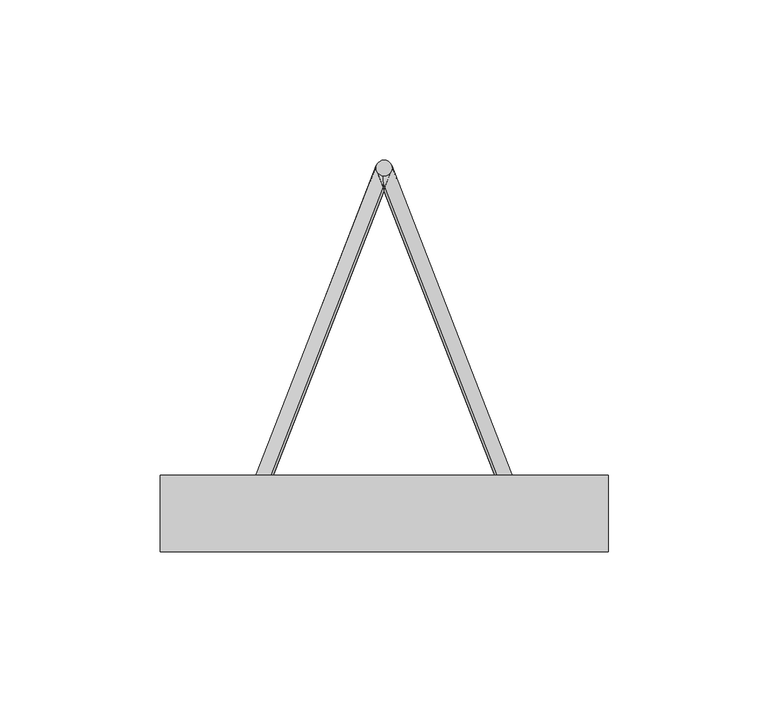
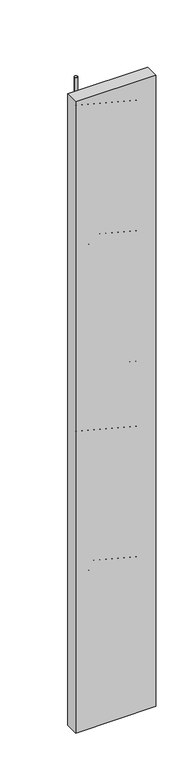
"""IFC4 building model written with IfcOpenShell, lengths in millimetres: proxy geometry, Vigota 3 (Pano 8) (Mf = 30)."""

from ifc_helpers import new_model, si_unit, point, frame, frame_2d, origin, origin_with_axes, origin_2d, place, context, project, spatial, polyline, circle_curve, trimmed, segment, composite_curve, outline, extrude, source, transform, mapped, element, save


def structural_framing_a67fc522(model_context):
    return source(origin(), model_context, "Body", "SweptSolid", [
        extrude(outline(polyline([(-70.0, 12.0), (70.0, 12.0), (70.0, -12.0), (-70.0, -12.0), (-70.0, 12.0)])), origin_with_axes(), (0.0, 0.0, 1.0), 1161.691264),
        extrude(outline(composite_curve([segment(trimmed(circle_curve(frame_2d((42.0, 0.0)), 2.5), [point((44.5, 0.0))], [point((39.5, 0.0))], False, "CARTESIAN"), True, "CONTINUOUS"), segment(trimmed(circle_curve(frame_2d((42.0, 0.0)), 2.5), [point((39.5, 0.0))], [point((44.5, 0.0))], False, "CARTESIAN"), True, "CONTINUOUS")], self_intersect=False)), frame((0.0, 0.0, 28.0), z_axis=(0.0, 0.0, 1.0), x_axis=(1.0, 0.0, 0.0)), (0.0, 0.0, 1.0), 1105.691264),
        extrude(outline(composite_curve([segment(trimmed(circle_curve(frame_2d((0.0, 108.0)), 2.5), [point((2.5, 108.0))], [point((-2.5, 108.0))], False, "CARTESIAN"), True, "CONTINUOUS"), segment(trimmed(circle_curve(frame_2d((0.0, 108.0)), 2.5), [point((-2.5, 108.0))], [point((2.5, 108.0))], False, "CARTESIAN"), True, "CONTINUOUS")], self_intersect=False)), frame((0.0, 0.0, 50.8456318), z_axis=(0.0, 0.0, 1.0), x_axis=(1.0, 0.0, 0.0)), (0.0, 0.0, 1.0), 1060.0),
        extrude(outline(composite_curve([segment(trimmed(circle_curve(origin_2d(), 2.5), [point((2.5, 0.0))], [point((-2.5, 0.0))], False, "CARTESIAN"), True, "CONTINUOUS"), segment(trimmed(circle_curve(origin_2d(), 2.5), [point((-2.5, 0.0))], [point((2.5, 0.0))], False, "CARTESIAN"), True, "CONTINUOUS")], self_intersect=False)), frame((42.0, 0.0, 40.8456318), z_axis=(-0.3218603428886276, 0.8276408817707567, 0.4598004898837537), x_axis=(0.8192319205108605, -3.936835275445103e-11, 0.5734623443750141)), (0.0, 0.0, 1.0), 130.491379),
        extrude(outline(composite_curve([segment(trimmed(circle_curve(origin_2d(), 2.5), [point((2.5, 0.0))], [point((-2.5, 0.0))], False, "CARTESIAN"), True, "CONTINUOUS"), segment(trimmed(circle_curve(origin_2d(), 2.5), [point((-2.5, 0.0))], [point((2.5, 0.0))], False, "CARTESIAN"), True, "CONTINUOUS")], self_intersect=False)), frame((0.0, 108.0, 100.8456318), z_axis=(0.3218603428886276, -0.8276408817707567, 0.4598004898837537), x_axis=(0.8192319205108605, -3.936835275445103e-11, -0.5734623443750141)), (0.0, 0.0, 1.0), 130.491379),
        extrude(outline(composite_curve([segment(trimmed(circle_curve(origin_2d(), 2.5), [point((2.5, 0.0))], [point((-2.5, 0.0))], False, "CARTESIAN"), True, "CONTINUOUS"), segment(trimmed(circle_curve(origin_2d(), 2.5), [point((-2.5, 0.0))], [point((2.5, 0.0))], False, "CARTESIAN"), True, "CONTINUOUS")], self_intersect=False)), frame((42.0, 0.0, 160.8456318), z_axis=(-0.3218603428886276, 0.8276408817707567, 0.4598004898837537), x_axis=(0.8192319205108605, -3.936835275445103e-11, 0.5734623443750141)), (0.0, 0.0, 1.0), 130.491379),
        extrude(outline(composite_curve([segment(trimmed(circle_curve(origin_2d(), 2.5), [point((2.5, 0.0))], [point((-2.5, 0.0))], False, "CARTESIAN"), True, "CONTINUOUS"), segment(trimmed(circle_curve(origin_2d(), 2.5), [point((-2.5, 0.0))], [point((2.5, 0.0))], False, "CARTESIAN"), True, "CONTINUOUS")], self_intersect=False)), frame((0.0, 108.0, 220.8456318), z_axis=(0.3218603428886276, -0.8276408817707567, 0.4598004898837537), x_axis=(0.8192319205108605, -3.936835275445103e-11, -0.5734623443750141)), (0.0, 0.0, 1.0), 130.491379),
        extrude(outline(composite_curve([segment(trimmed(circle_curve(origin_2d(), 2.5), [point((2.5, 0.0))], [point((-2.5, 0.0))], False, "CARTESIAN"), True, "CONTINUOUS"), segment(trimmed(circle_curve(origin_2d(), 2.5), [point((-2.5, 0.0))], [point((2.5, 0.0))], False, "CARTESIAN"), True, "CONTINUOUS")], self_intersect=False)), frame((42.0, 0.0, 280.8456318), z_axis=(-0.3218603428886276, 0.8276408817707567, 0.4598004898837537), x_axis=(0.8192319205108605, -3.936835275445103e-11, 0.5734623443750141)), (0.0, 0.0, 1.0), 130.491379),
        extrude(outline(composite_curve([segment(trimmed(circle_curve(origin_2d(), 2.5), [point((2.5, 0.0))], [point((-2.5, 0.0))], False, "CARTESIAN"), True, "CONTINUOUS"), segment(trimmed(circle_curve(origin_2d(), 2.5), [point((-2.5, 0.0))], [point((2.5, 0.0))], False, "CARTESIAN"), True, "CONTINUOUS")], self_intersect=False)), frame((0.0, 108.0, 340.8456318), z_axis=(0.3218603428886276, -0.8276408817707567, 0.4598004898837537), x_axis=(0.8192319205108605, -3.936835275445103e-11, -0.5734623443750141)), (0.0, 0.0, 1.0), 130.491379),
        extrude(outline(composite_curve([segment(trimmed(circle_curve(origin_2d(), 2.5), [point((2.5, 0.0))], [point((-2.5, 0.0))], False, "CARTESIAN"), True, "CONTINUOUS"), segment(trimmed(circle_curve(origin_2d(), 2.5), [point((-2.5, 0.0))], [point((2.5, 0.0))], False, "CARTESIAN"), True, "CONTINUOUS")], self_intersect=False)), frame((42.0, 0.0, 400.8456318), z_axis=(-0.3218603428886276, 0.8276408817707567, 0.4598004898837537), x_axis=(0.8192319205108605, -3.936835275445103e-11, 0.5734623443750141)), (0.0, 0.0, 1.0), 130.491379),
        extrude(outline(composite_curve([segment(trimmed(circle_curve(origin_2d(), 2.5), [point((2.5, 0.0))], [point((-2.5, 0.0))], False, "CARTESIAN"), True, "CONTINUOUS"), segment(trimmed(circle_curve(origin_2d(), 2.5), [point((-2.5, 0.0))], [point((2.5, 0.0))], False, "CARTESIAN"), True, "CONTINUOUS")], self_intersect=False)), frame((0.0, 108.0, 460.8456318), z_axis=(0.3218603428886276, -0.8276408817707567, 0.4598004898837537), x_axis=(0.8192319205108605, -3.936835275445103e-11, -0.5734623443750141)), (0.0, 0.0, 1.0), 130.491379),
        extrude(outline(composite_curve([segment(trimmed(circle_curve(origin_2d(), 2.5), [point((2.5, 0.0))], [point((-2.5, 0.0))], False, "CARTESIAN"), True, "CONTINUOUS"), segment(trimmed(circle_curve(origin_2d(), 2.5), [point((-2.5, 0.0))], [point((2.5, 0.0))], False, "CARTESIAN"), True, "CONTINUOUS")], self_intersect=False)), frame((42.0, 0.0, 520.8456318), z_axis=(-0.3218603428886276, 0.8276408817707567, 0.4598004898837537), x_axis=(0.8192319205108605, -3.936835275445103e-11, 0.5734623443750141)), (0.0, 0.0, 1.0), 130.491379),
        extrude(outline(composite_curve([segment(trimmed(circle_curve(origin_2d(), 2.5), [point((2.5, 0.0))], [point((-2.5, 0.0))], False, "CARTESIAN"), True, "CONTINUOUS"), segment(trimmed(circle_curve(origin_2d(), 2.5), [point((-2.5, 0.0))], [point((2.5, 0.0))], False, "CARTESIAN"), True, "CONTINUOUS")], self_intersect=False)), frame((0.0, 108.0, 580.8456318), z_axis=(0.3218603428886276, -0.8276408817707567, 0.4598004898837537), x_axis=(0.8192319205108605, -3.936835275445103e-11, -0.5734623443750141)), (0.0, 0.0, 1.0), 130.491379),
        extrude(outline(composite_curve([segment(trimmed(circle_curve(origin_2d(), 2.5), [point((2.5, 0.0))], [point((-2.5, 0.0))], False, "CARTESIAN"), True, "CONTINUOUS"), segment(trimmed(circle_curve(origin_2d(), 2.5), [point((-2.5, 0.0))], [point((2.5, 0.0))], False, "CARTESIAN"), True, "CONTINUOUS")], self_intersect=False)), frame((42.0, 0.0, 640.8456318), z_axis=(-0.3218603428886276, 0.8276408817707567, 0.4598004898837537), x_axis=(0.8192319205108605, -3.936835275445103e-11, 0.5734623443750141)), (0.0, 0.0, 1.0), 130.491379),
        extrude(outline(composite_curve([segment(trimmed(circle_curve(origin_2d(), 2.5), [point((2.5, 0.0))], [point((-2.5, 0.0))], False, "CARTESIAN"), True, "CONTINUOUS"), segment(trimmed(circle_curve(origin_2d(), 2.5), [point((-2.5, 0.0))], [point((2.5, 0.0))], False, "CARTESIAN"), True, "CONTINUOUS")], self_intersect=False)), frame((0.0, 108.0, 700.8456318), z_axis=(0.3218603428886276, -0.8276408817707567, 0.4598004898837537), x_axis=(0.8192319205108605, -3.936835275445103e-11, -0.5734623443750141)), (0.0, 0.0, 1.0), 130.491379),
        extrude(outline(composite_curve([segment(trimmed(circle_curve(origin_2d(), 2.5), [point((2.5, 0.0))], [point((-2.5, 0.0))], False, "CARTESIAN"), True, "CONTINUOUS"), segment(trimmed(circle_curve(origin_2d(), 2.5), [point((-2.5, 0.0))], [point((2.5, 0.0))], False, "CARTESIAN"), True, "CONTINUOUS")], self_intersect=False)), frame((42.0, 0.0, 760.8456318), z_axis=(-0.3218603428886276, 0.8276408817707567, 0.4598004898837537), x_axis=(0.8192319205108605, -3.936835275445103e-11, 0.5734623443750141)), (0.0, 0.0, 1.0), 130.491379),
        extrude(outline(composite_curve([segment(trimmed(circle_curve(origin_2d(), 2.5), [point((2.5, 0.0))], [point((-2.5, 0.0))], False, "CARTESIAN"), True, "CONTINUOUS"), segment(trimmed(circle_curve(origin_2d(), 2.5), [point((-2.5, 0.0))], [point((2.5, 0.0))], False, "CARTESIAN"), True, "CONTINUOUS")], self_intersect=False)), frame((0.0, 108.0, 820.8456318), z_axis=(0.3218603428886276, -0.8276408817707567, 0.4598004898837537), x_axis=(0.8192319205108605, -3.936835275445103e-11, -0.5734623443750141)), (0.0, 0.0, 1.0), 130.491379),
        extrude(outline(composite_curve([segment(trimmed(circle_curve(origin_2d(), 2.5), [point((2.5, 0.0))], [point((-2.5, 0.0))], False, "CARTESIAN"), True, "CONTINUOUS"), segment(trimmed(circle_curve(origin_2d(), 2.5), [point((-2.5, 0.0))], [point((2.5, 0.0))], False, "CARTESIAN"), True, "CONTINUOUS")], self_intersect=False)), frame((42.0, 0.0, 880.8456318), z_axis=(-0.3218603428886276, 0.8276408817707567, 0.4598004898837537), x_axis=(0.8192319205108605, -3.936835275445103e-11, 0.5734623443750141)), (0.0, 0.0, 1.0), 130.491379),
        extrude(outline(composite_curve([segment(trimmed(circle_curve(origin_2d(), 2.5), [point((2.5, 0.0))], [point((-2.5, 0.0))], False, "CARTESIAN"), True, "CONTINUOUS"), segment(trimmed(circle_curve(origin_2d(), 2.5), [point((-2.5, 0.0))], [point((2.5, 0.0))], False, "CARTESIAN"), True, "CONTINUOUS")], self_intersect=False)), frame((0.0, 108.0, 940.8456318), z_axis=(0.3218603428886276, -0.8276408817707567, 0.4598004898837537), x_axis=(0.8192319205108605, -3.936835275445103e-11, -0.5734623443750141)), (0.0, 0.0, 1.0), 130.491379),
        extrude(outline(composite_curve([segment(trimmed(circle_curve(origin_2d(), 2.5), [point((2.5, 0.0))], [point((-2.5, 0.0))], False, "CARTESIAN"), True, "CONTINUOUS"), segment(trimmed(circle_curve(origin_2d(), 2.5), [point((-2.5, 0.0))], [point((2.5, 0.0))], False, "CARTESIAN"), True, "CONTINUOUS")], self_intersect=False)), frame((42.0, 0.0, 1000.8456318), z_axis=(-0.3218603428886276, 0.8276408817707567, 0.4598004898837537), x_axis=(0.8192319205108605, -3.936835275445103e-11, 0.5734623443750141)), (0.0, 0.0, 1.0), 130.491379),
        extrude(outline(composite_curve([segment(trimmed(circle_curve(origin_2d(), 2.5), [point((2.5, 0.0))], [point((-2.5, 0.0))], False, "CARTESIAN"), True, "CONTINUOUS"), segment(trimmed(circle_curve(origin_2d(), 2.5), [point((-2.5, 0.0))], [point((2.5, 0.0))], False, "CARTESIAN"), True, "CONTINUOUS")], self_intersect=False)), frame((0.0, 108.0, 1060.845632), z_axis=(0.3218603428886276, -0.8276408817707567, 0.4598004898837537), x_axis=(0.8192319205108605, -3.936835275445103e-11, -0.5734623443750141)), (0.0, 0.0, 1.0), 130.491379),
        extrude(outline(composite_curve([segment(trimmed(circle_curve(frame_2d((-42.0, 0.0)), 2.5), [point((-39.5, 0.0))], [point((-44.5, 0.0))], False, "CARTESIAN"), True, "CONTINUOUS"), segment(trimmed(circle_curve(frame_2d((-42.0, 0.0)), 2.5), [point((-44.5, 0.0))], [point((-39.5, 0.0))], False, "CARTESIAN"), True, "CONTINUOUS")], self_intersect=False)), frame((0.0, 0.0, 28.0), z_axis=(0.0, 0.0, 1.0), x_axis=(1.0, 0.0, 0.0)), (0.0, 0.0, 1.0), 1105.691264),
        extrude(outline(composite_curve([segment(trimmed(circle_curve(origin_2d(), 2.5), [point((2.5, 0.0))], [point((-2.5, 0.0))], False, "CARTESIAN"), True, "CONTINUOUS"), segment(trimmed(circle_curve(origin_2d(), 2.5), [point((-2.5, 0.0))], [point((2.5, 0.0))], False, "CARTESIAN"), True, "CONTINUOUS")], self_intersect=False)), frame((-42.0, 0.0, 40.8456318), z_axis=(0.3218603428886276, 0.8276408817707567, 0.4598004898837537), x_axis=(0.8192319205108605, 3.936835275445103e-11, -0.5734623443750141)), (0.0, 0.0, 1.0), 130.491379),
        extrude(outline(composite_curve([segment(trimmed(circle_curve(origin_2d(), 2.5), [point((2.5, 0.0))], [point((-2.5, 0.0))], False, "CARTESIAN"), True, "CONTINUOUS"), segment(trimmed(circle_curve(origin_2d(), 2.5), [point((-2.5, 0.0))], [point((2.5, 0.0))], False, "CARTESIAN"), True, "CONTINUOUS")], self_intersect=False)), frame((0.0, 108.0, 100.8456318), z_axis=(-0.3218603428886276, -0.8276408817707567, 0.4598004898837537), x_axis=(0.8192319205108605, 3.936835275445103e-11, 0.5734623443750141)), (0.0, 0.0, 1.0), 130.491379),
        extrude(outline(composite_curve([segment(trimmed(circle_curve(origin_2d(), 2.5), [point((2.5, 0.0))], [point((-2.5, 0.0))], False, "CARTESIAN"), True, "CONTINUOUS"), segment(trimmed(circle_curve(origin_2d(), 2.5), [point((-2.5, 0.0))], [point((2.5, 0.0))], False, "CARTESIAN"), True, "CONTINUOUS")], self_intersect=False)), frame((-42.0, 0.0, 160.8456318), z_axis=(0.3218603428886276, 0.8276408817707567, 0.4598004898837537), x_axis=(0.8192319205108605, 3.936835275445103e-11, -0.5734623443750141)), (0.0, 0.0, 1.0), 130.491379),
        extrude(outline(composite_curve([segment(trimmed(circle_curve(origin_2d(), 2.5), [point((2.5, 0.0))], [point((-2.5, 0.0))], False, "CARTESIAN"), True, "CONTINUOUS"), segment(trimmed(circle_curve(origin_2d(), 2.5), [point((-2.5, 0.0))], [point((2.5, 0.0))], False, "CARTESIAN"), True, "CONTINUOUS")], self_intersect=False)), frame((0.0, 108.0, 220.8456318), z_axis=(-0.3218603428886276, -0.8276408817707567, 0.4598004898837537), x_axis=(0.8192319205108605, 3.936835275445103e-11, 0.5734623443750141)), (0.0, 0.0, 1.0), 130.491379),
        extrude(outline(composite_curve([segment(trimmed(circle_curve(origin_2d(), 2.5), [point((2.5, 0.0))], [point((-2.5, 0.0))], False, "CARTESIAN"), True, "CONTINUOUS"), segment(trimmed(circle_curve(origin_2d(), 2.5), [point((-2.5, 0.0))], [point((2.5, 0.0))], False, "CARTESIAN"), True, "CONTINUOUS")], self_intersect=False)), frame((-42.0, 0.0, 280.8456318), z_axis=(0.3218603428886276, 0.8276408817707567, 0.4598004898837537), x_axis=(0.8192319205108605, 3.936835275445103e-11, -0.5734623443750141)), (0.0, 0.0, 1.0), 130.491379),
        extrude(outline(composite_curve([segment(trimmed(circle_curve(origin_2d(), 2.5), [point((2.5, 0.0))], [point((-2.5, 0.0))], False, "CARTESIAN"), True, "CONTINUOUS"), segment(trimmed(circle_curve(origin_2d(), 2.5), [point((-2.5, 0.0))], [point((2.5, 0.0))], False, "CARTESIAN"), True, "CONTINUOUS")], self_intersect=False)), frame((0.0, 108.0, 340.8456318), z_axis=(-0.3218603428886276, -0.8276408817707567, 0.4598004898837537), x_axis=(0.8192319205108605, 3.936835275445103e-11, 0.5734623443750141)), (0.0, 0.0, 1.0), 130.491379),
        extrude(outline(composite_curve([segment(trimmed(circle_curve(origin_2d(), 2.5), [point((2.5, 0.0))], [point((-2.5, 0.0))], False, "CARTESIAN"), True, "CONTINUOUS"), segment(trimmed(circle_curve(origin_2d(), 2.5), [point((-2.5, 0.0))], [point((2.5, 0.0))], False, "CARTESIAN"), True, "CONTINUOUS")], self_intersect=False)), frame((-42.0, 0.0, 400.8456318), z_axis=(0.3218603428886276, 0.8276408817707567, 0.4598004898837537), x_axis=(0.8192319205108605, 3.936835275445103e-11, -0.5734623443750141)), (0.0, 0.0, 1.0), 130.491379),
        extrude(outline(composite_curve([segment(trimmed(circle_curve(origin_2d(), 2.5), [point((2.5, 0.0))], [point((-2.5, 0.0))], False, "CARTESIAN"), True, "CONTINUOUS"), segment(trimmed(circle_curve(origin_2d(), 2.5), [point((-2.5, 0.0))], [point((2.5, 0.0))], False, "CARTESIAN"), True, "CONTINUOUS")], self_intersect=False)), frame((0.0, 108.0, 460.8456318), z_axis=(-0.3218603428886276, -0.8276408817707567, 0.4598004898837537), x_axis=(0.8192319205108605, 3.936835275445103e-11, 0.5734623443750141)), (0.0, 0.0, 1.0), 130.491379),
        extrude(outline(composite_curve([segment(trimmed(circle_curve(origin_2d(), 2.5), [point((2.5, 0.0))], [point((-2.5, 0.0))], False, "CARTESIAN"), True, "CONTINUOUS"), segment(trimmed(circle_curve(origin_2d(), 2.5), [point((-2.5, 0.0))], [point((2.5, 0.0))], False, "CARTESIAN"), True, "CONTINUOUS")], self_intersect=False)), frame((-42.0, 0.0, 520.8456318), z_axis=(0.3218603428886276, 0.8276408817707567, 0.4598004898837537), x_axis=(0.8192319205108605, 3.936835275445103e-11, -0.5734623443750141)), (0.0, 0.0, 1.0), 130.491379),
        extrude(outline(composite_curve([segment(trimmed(circle_curve(origin_2d(), 2.5), [point((2.5, 0.0))], [point((-2.5, 0.0))], False, "CARTESIAN"), True, "CONTINUOUS"), segment(trimmed(circle_curve(origin_2d(), 2.5), [point((-2.5, 0.0))], [point((2.5, 0.0))], False, "CARTESIAN"), True, "CONTINUOUS")], self_intersect=False)), frame((0.0, 108.0, 580.8456318), z_axis=(-0.3218603428886276, -0.8276408817707567, 0.4598004898837537), x_axis=(0.8192319205108605, 3.936835275445103e-11, 0.5734623443750141)), (0.0, 0.0, 1.0), 130.491379),
        extrude(outline(composite_curve([segment(trimmed(circle_curve(origin_2d(), 2.5), [point((2.5, 0.0))], [point((-2.5, 0.0))], False, "CARTESIAN"), True, "CONTINUOUS"), segment(trimmed(circle_curve(origin_2d(), 2.5), [point((-2.5, 0.0))], [point((2.5, 0.0))], False, "CARTESIAN"), True, "CONTINUOUS")], self_intersect=False)), frame((-42.0, 0.0, 640.8456318), z_axis=(0.3218603428886276, 0.8276408817707567, 0.4598004898837537), x_axis=(0.8192319205108605, 3.936835275445103e-11, -0.5734623443750141)), (0.0, 0.0, 1.0), 130.491379),
        extrude(outline(composite_curve([segment(trimmed(circle_curve(origin_2d(), 2.5), [point((2.5, 0.0))], [point((-2.5, 0.0))], False, "CARTESIAN"), True, "CONTINUOUS"), segment(trimmed(circle_curve(origin_2d(), 2.5), [point((-2.5, 0.0))], [point((2.5, 0.0))], False, "CARTESIAN"), True, "CONTINUOUS")], self_intersect=False)), frame((0.0, 108.0, 700.8456318), z_axis=(-0.3218603428886276, -0.8276408817707567, 0.4598004898837537), x_axis=(0.8192319205108605, 3.936835275445103e-11, 0.5734623443750141)), (0.0, 0.0, 1.0), 130.491379),
        extrude(outline(composite_curve([segment(trimmed(circle_curve(origin_2d(), 2.5), [point((2.5, 0.0))], [point((-2.5, 0.0))], False, "CARTESIAN"), True, "CONTINUOUS"), segment(trimmed(circle_curve(origin_2d(), 2.5), [point((-2.5, 0.0))], [point((2.5, 0.0))], False, "CARTESIAN"), True, "CONTINUOUS")], self_intersect=False)), frame((-42.0, 0.0, 760.8456318), z_axis=(0.3218603428886276, 0.8276408817707567, 0.4598004898837537), x_axis=(0.8192319205108605, 3.936835275445103e-11, -0.5734623443750141)), (0.0, 0.0, 1.0), 130.491379),
        extrude(outline(composite_curve([segment(trimmed(circle_curve(origin_2d(), 2.5), [point((2.5, 0.0))], [point((-2.5, 0.0))], False, "CARTESIAN"), True, "CONTINUOUS"), segment(trimmed(circle_curve(origin_2d(), 2.5), [point((-2.5, 0.0))], [point((2.5, 0.0))], False, "CARTESIAN"), True, "CONTINUOUS")], self_intersect=False)), frame((0.0, 108.0, 820.8456318), z_axis=(-0.3218603428886276, -0.8276408817707567, 0.4598004898837537), x_axis=(0.8192319205108605, 3.936835275445103e-11, 0.5734623443750141)), (0.0, 0.0, 1.0), 130.491379),
        extrude(outline(composite_curve([segment(trimmed(circle_curve(origin_2d(), 2.5), [point((2.5, 0.0))], [point((-2.5, 0.0))], False, "CARTESIAN"), True, "CONTINUOUS"), segment(trimmed(circle_curve(origin_2d(), 2.5), [point((-2.5, 0.0))], [point((2.5, 0.0))], False, "CARTESIAN"), True, "CONTINUOUS")], self_intersect=False)), frame((-42.0, 0.0, 880.8456318), z_axis=(0.3218603428886276, 0.8276408817707567, 0.4598004898837537), x_axis=(0.8192319205108605, 3.936835275445103e-11, -0.5734623443750141)), (0.0, 0.0, 1.0), 130.491379),
        extrude(outline(composite_curve([segment(trimmed(circle_curve(origin_2d(), 2.5), [point((2.5, 0.0))], [point((-2.5, 0.0))], False, "CARTESIAN"), True, "CONTINUOUS"), segment(trimmed(circle_curve(origin_2d(), 2.5), [point((-2.5, 0.0))], [point((2.5, 0.0))], False, "CARTESIAN"), True, "CONTINUOUS")], self_intersect=False)), frame((0.0, 108.0, 940.8456318), z_axis=(-0.3218603428886276, -0.8276408817707567, 0.4598004898837537), x_axis=(0.8192319205108605, 3.936835275445103e-11, 0.5734623443750141)), (0.0, 0.0, 1.0), 130.491379),
        extrude(outline(composite_curve([segment(trimmed(circle_curve(origin_2d(), 2.5), [point((2.5, 0.0))], [point((-2.5, 0.0))], False, "CARTESIAN"), True, "CONTINUOUS"), segment(trimmed(circle_curve(origin_2d(), 2.5), [point((-2.5, 0.0))], [point((2.5, 0.0))], False, "CARTESIAN"), True, "CONTINUOUS")], self_intersect=False)), frame((-42.0, 0.0, 1000.8456318), z_axis=(0.3218603428886276, 0.8276408817707567, 0.4598004898837537), x_axis=(0.8192319205108605, 3.936835275445103e-11, -0.5734623443750141)), (0.0, 0.0, 1.0), 130.491379),
        extrude(outline(composite_curve([segment(trimmed(circle_curve(origin_2d(), 2.5), [point((2.5, 0.0))], [point((-2.5, 0.0))], False, "CARTESIAN"), True, "CONTINUOUS"), segment(trimmed(circle_curve(origin_2d(), 2.5), [point((-2.5, 0.0))], [point((2.5, 0.0))], False, "CARTESIAN"), True, "CONTINUOUS")], self_intersect=False)), frame((0.0, 108.0, 1060.845632), z_axis=(-0.3218603428886276, -0.8276408817707567, 0.4598004898837537), x_axis=(0.8192319205108605, 3.936835275445103e-11, 0.5734623443750141)), (0.0, 0.0, 1.0), 130.491379),
    ])


if __name__ == "__main__":
    model = new_model("IFC4")
    model_context = context("Model", 3, world=origin())
    ifc_project = project(units=[si_unit("LENGTHUNIT", "METRE", prefix="MILLI")], contexts=[model_context])
    site = spatial("IfcSite", under=ifc_project)
    building = spatial("IfcBuilding", under=site)
    placement = place(None, origin())
    structural_framing_shape = structural_framing_a67fc522(model_context)
    element("IfcBuildingElementProxy", 1, Name="Vigota 3 (Pano 8) (Mf = 30)", ObjectType="Vigota 3 (Pano 8) (Mf = 30)", at=placement, inside=building, context=model_context, shape_type="MappedRepresentation", body=[
        mapped(structural_framing_shape, transform((0.0, 0.0, 0.0), x_axis=(1.0, 0.0, 0.0), y_axis=(0.0, 1.0, 0.0), z_axis=(0.0, 0.0, 1.0))),
    ])
    save(model, "model.ifc")

# Revit data of these elements
# Element 1 (IfcBuildingElementProxy, "Vigota 3 (Pano 8) (Mf = 30)")
#   Materials on its faces: "Aço", "Concreto armado"
# Materials
#   "Aço": class "Metal", colour RGB 120 120 120, transparency 0, Description = "Aço estrutural A36 grau, ASTM B, acabamento laminado", Cost = 0
#   "Concreto armado": class "Não atribuído", colour RGB 168 169 158, transparency 0
